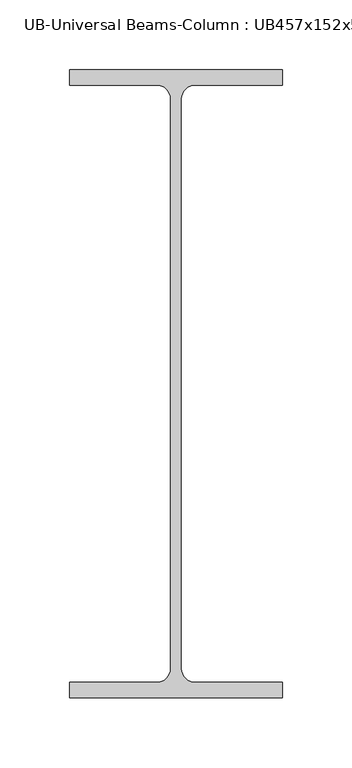
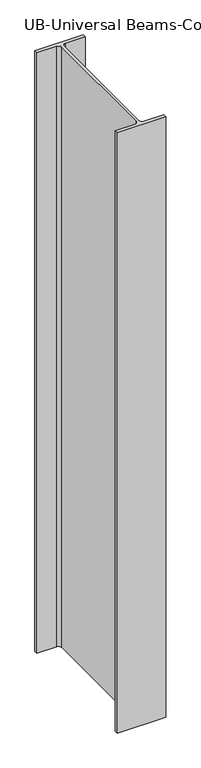
"""IFC4 building model written with IfcOpenShell, lengths in millimetres: column geometry, UB-Universal Beams-Column : UB457x152x52."""

from ifc_helpers import new_model, si_unit, point, frame_2d, origin, origin_with_axes, place, context, project, spatial, polyline, circle_curve, trimmed, segment, composite_curve, outline, extrude, source, transform, mapped, element, save


def ub_universal_beams_column_ub457x152x52_1aa4cf6f(model_context):
    return source(origin(), model_context, "Body", "SweptSolid", [
        extrude(outline(composite_curve([segment(polyline([(76.2, 224.9), (76.2, 214.0), (14.0, 214.0)]), True, "CONTINUOUS"), segment(trimmed(circle_curve(frame_2d((14.0, 203.8)), 10.2), [point((14.0, 214.0))], [point((3.8, 203.8))], True, "CARTESIAN"), True, "CONTINUOUS"), segment(polyline([(3.8, 203.8), (3.8, -203.8)]), True, "CONTINUOUS"), segment(trimmed(circle_curve(frame_2d((14.0, -203.8)), 10.2), [point((3.8, -203.8))], [point((14.0, -214.0))], True, "CARTESIAN"), True, "CONTINUOUS"), segment(polyline([(14.0, -214.0), (76.2, -214.0), (76.2, -224.9), (-76.2, -224.9), (-76.2, -214.0), (-14.0, -214.0)]), True, "CONTINUOUS"), segment(trimmed(circle_curve(frame_2d((-14.0, -203.8)), 10.2), [point((-14.0, -214.0))], [point((-3.8, -203.8))], True, "CARTESIAN"), True, "CONTINUOUS"), segment(polyline([(-3.8, -203.8), (-3.8, 203.8)]), True, "CONTINUOUS"), segment(trimmed(circle_curve(frame_2d((-14.0, 203.8)), 10.2), [point((-3.8, 203.8))], [point((-14.0, 214.0))], True, "CARTESIAN"), True, "CONTINUOUS"), segment(polyline([(-14.0, 214.0), (-76.2, 214.0), (-76.2, 224.9), (76.2, 224.9)]), True, "CONTINUOUS")], self_intersect=False)), origin_with_axes(), (0.0, 0.0, 1.0), 2000.0),
    ])


if __name__ == "__main__":
    model = new_model("IFC4")
    model_context = context("Model", 3, world=origin())
    ifc_project = project(units=[si_unit("LENGTHUNIT", "METRE", prefix="MILLI")], contexts=[model_context])
    site = spatial("IfcSite", under=ifc_project)
    building = spatial("IfcBuilding", under=site)
    placement = place(None, origin())
    ub_universal_beams_column_ub457x152x52_shape = ub_universal_beams_column_ub457x152x52_1aa4cf6f(model_context)
    element("IfcColumn", 1, ObjectType="UB-Universal Beams-Column : UB457x152x52", at=placement, inside=building, context=model_context, shape_type="MappedRepresentation", body=[
        mapped(ub_universal_beams_column_ub457x152x52_shape, transform((0.0, 0.0, 0.0), x_axis=(1.0, 0.0, 0.0), y_axis=(0.0, 1.0, 0.0), z_axis=(0.0, 0.0, 1.0))),
    ])
    save(model, "model.ifc")

# Revit data of these elements
# Type "UB-Universal Beams-Column : UB457x152x52"
#   Section Name Key = "UB457X152X52"
#   Width = 15.24 cm
#   Web Thickness = 0.76 cm
#   Web Fillet = 1.02 cm
#   Warping Constant = 311000.0 cm⁶
#   Torsional Moment of Inertia = 21.40 cm⁴
#   Section Area = 66.6 cm²
#   Plastic Modulus weak axis = 133.0 cm³
#   Plastic Modulus strong axis = 1096.0 cm³
#   Nominal Weight = 52.2998 kgf/m
#   Moment of Inertia weak axis = 645.00 cm⁴
#   Moment of Inertia strong axis = 21369.00 cm⁴
#   Height = 44.98 cm
#   Flange Thickness = 1.09 cm
#   Elastic Modulus weak axis = 85.0 cm³
#   Elastic Modulus strong axis = 950.0 cm³
#   Centroid Vertical = 22.49 cm
#   Centroid Horizontal = 7.62 cm
#   Bolt Spacing = 9.0 cm
#   Structural Material [instance default] = Metal - Steel 43-275
#   Type Comments = ""
#   Assembly Code = ""
# Element 1 (IfcColumn, "UB-Universal Beams-Column : UB457x152x52")
#   Materials on its faces: "Metal - Steel 43-275"
# Materials
#   "Metal - Steel 43-275": class "Metal", colour RGB 247 247 247, transparency 0, Cost = 0
